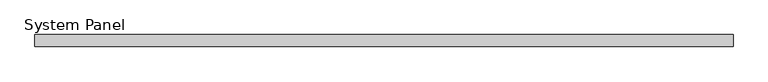
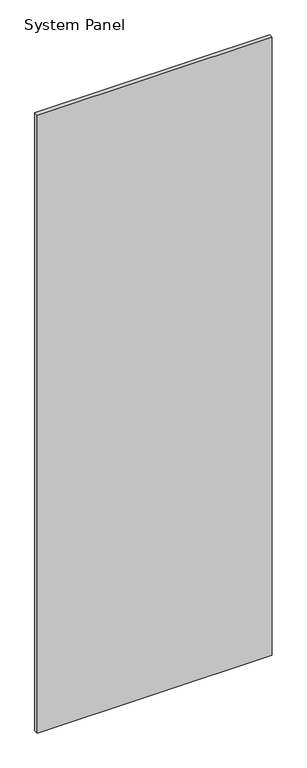
"""IFC4 building model written with IfcOpenShell, lengths in millimetres: plate geometry, System Panel : WWm-Glass-20mm-10mmOffset."""

from ifc_helpers import new_model, si_unit, origin, origin_with_axes, place, context, project, spatial, polyline, outline, extrude, source, transform, mapped, element, save


def system_panel_89065135(model_context):
    return source(origin(), model_context, "Body", "SweptSolid", [
        extrude(outline(polyline([(585.0, 0.0), (-585.0, 0.0), (-585.0, 20.0), (585.0, 20.0), (585.0, 0.0)])), origin_with_axes(), (0.0, 0.0, 1.0), 3250.0),
    ])


if __name__ == "__main__":
    model = new_model("IFC4")
    model_context = context("Model", 3, world=origin())
    ifc_project = project(units=[si_unit("LENGTHUNIT", "METRE", prefix="MILLI")], contexts=[model_context])
    site = spatial("IfcSite", under=ifc_project)
    building = spatial("IfcBuilding", under=site)
    placement = place(None, origin())
    system_panel_shape = system_panel_89065135(model_context)
    element("IfcPlate", 1, ObjectType="System Panel : WWm-Glass-20mm-10mmOffset", at=placement, inside=building, context=model_context, shape_type="MappedRepresentation", body=[
        mapped(system_panel_shape, transform((0.0, 0.0, 0.0), x_axis=(1.0, 0.0, 0.0), y_axis=(0.0, 1.0, 0.0), z_axis=(0.0, 0.0, 1.0))),
    ])
    save(model, "model.ifc")

# Revit data of these elements
# Type "System Panel : WWm-Glass-20mm-10mmOffset"
#   Finish = ""
# Element 1 (IfcPlate, "System Panel : WWm-Glass-20mm-10mmOffset")
#   Materials on its faces: "WW-EC-GL-Storefront"
# Materials
#   "WW-EC-GL-Storefront": class "Glass", colour RGB 236 240 239, transparency 0.85, Description = "Storefront Glass", Cost = 0
